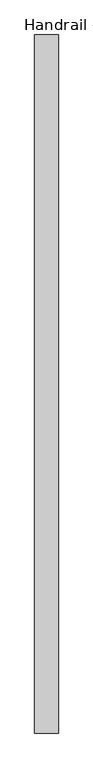
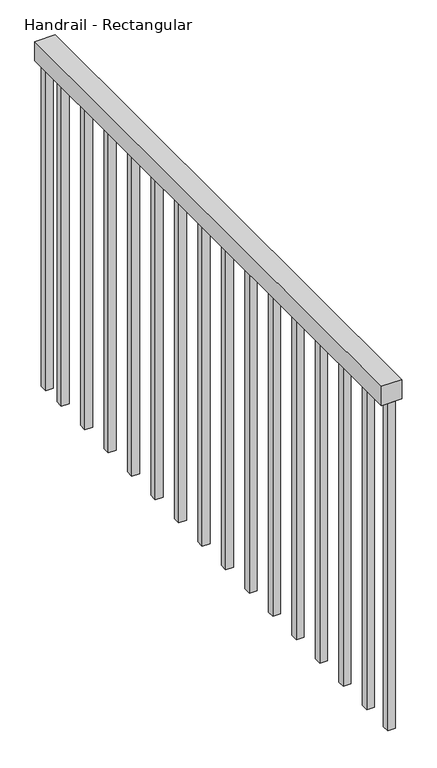
"""IFC4 building model written with IfcOpenShell, lengths in millimetres: railing geometry, Handrail - Rectangular."""

from ifc_helpers import new_model, si_unit, frame, origin, place, context, project, spatial, polyline, outline, extrude, source, transform, mapped, element, save


def handrail_rectangular_a0f4db76(model_context):
    return source(origin(), model_context, "Body", "SweptSolid", [
        extrude(outline(polyline([(-12364.4211091, 3845.8507146), (-12415.2211091, 3845.8507146), (-12415.2211091, 5345.8507146), (-12364.4211091, 5345.8507146), (-12364.4211091, 3845.8507146)])), frame((0.0, 0.0, 6654.4), z_axis=(0.0, 0.0, 1.0), x_axis=(1.0, 0.0, 0.0)), (0.0, 0.0, 1.0), 50.8),
        extrude(outline(polyline([(-12380.2961091, 5258.7257146), (-12399.3461091, 5258.7257146), (-12399.3461091, 5277.7757146), (-12380.2961091, 5277.7757146), (-12380.2961091, 5258.7257146)])), frame((0.0, 0.0, 5790.8), z_axis=(0.0, 0.0, 1.0), x_axis=(1.0, 0.0, 0.0)), (0.0, 0.0, 1.0), 863.6),
        extrude(outline(polyline([(-12380.2961091, 5157.1257146), (-12399.3461091, 5157.1257146), (-12399.3461091, 5176.1757146), (-12380.2961091, 5176.1757146), (-12380.2961091, 5157.1257146)])), frame((0.0, 0.0, 5790.8), z_axis=(0.0, 0.0, 1.0), x_axis=(1.0, 0.0, 0.0)), (0.0, 0.0, 1.0), 863.6),
        extrude(outline(polyline([(-12380.2961091, 5055.5257146), (-12399.3461091, 5055.5257146), (-12399.3461091, 5074.5757146), (-12380.2961091, 5074.5757146), (-12380.2961091, 5055.5257146)])), frame((0.0, 0.0, 5790.8), z_axis=(0.0, 0.0, 1.0), x_axis=(1.0, 0.0, 0.0)), (0.0, 0.0, 1.0), 863.6),
        extrude(outline(polyline([(-12380.2961091, 4953.9257146), (-12399.3461091, 4953.9257146), (-12399.3461091, 4972.9757146), (-12380.2961091, 4972.9757146), (-12380.2961091, 4953.9257146)])), frame((0.0, 0.0, 5790.8), z_axis=(0.0, 0.0, 1.0), x_axis=(1.0, 0.0, 0.0)), (0.0, 0.0, 1.0), 863.6),
        extrude(outline(polyline([(-12380.2961091, 4852.3257146), (-12399.3461091, 4852.3257146), (-12399.3461091, 4871.3757146), (-12380.2961091, 4871.3757146), (-12380.2961091, 4852.3257146)])), frame((0.0, 0.0, 5790.8), z_axis=(0.0, 0.0, 1.0), x_axis=(1.0, 0.0, 0.0)), (0.0, 0.0, 1.0), 863.6),
        extrude(outline(polyline([(-12380.2961091, 4750.7257146), (-12399.3461091, 4750.7257146), (-12399.3461091, 4769.7757146), (-12380.2961091, 4769.7757146), (-12380.2961091, 4750.7257146)])), frame((0.0, 0.0, 5790.8), z_axis=(0.0, 0.0, 1.0), x_axis=(1.0, 0.0, 0.0)), (0.0, 0.0, 1.0), 863.6),
        extrude(outline(polyline([(-12380.2961091, 4649.1257146), (-12399.3461091, 4649.1257146), (-12399.3461091, 4668.1757146), (-12380.2961091, 4668.1757146), (-12380.2961091, 4649.1257146)])), frame((0.0, 0.0, 5790.8), z_axis=(0.0, 0.0, 1.0), x_axis=(1.0, 0.0, 0.0)), (0.0, 0.0, 1.0), 863.6),
        extrude(outline(polyline([(-12380.2961091, 4547.5257146), (-12399.3461091, 4547.5257146), (-12399.3461091, 4566.5757146), (-12380.2961091, 4566.5757146), (-12380.2961091, 4547.5257146)])), frame((0.0, 0.0, 5790.8), z_axis=(0.0, 0.0, 1.0), x_axis=(1.0, 0.0, 0.0)), (0.0, 0.0, 1.0), 863.6),
        extrude(outline(polyline([(-12380.2961091, 4445.9257146), (-12399.3461091, 4445.9257146), (-12399.3461091, 4464.9757146), (-12380.2961091, 4464.9757146), (-12380.2961091, 4445.9257146)])), frame((0.0, 0.0, 5790.8), z_axis=(0.0, 0.0, 1.0), x_axis=(1.0, 0.0, 0.0)), (0.0, 0.0, 1.0), 863.6),
        extrude(outline(polyline([(-12380.2961091, 4344.3257146), (-12399.3461091, 4344.3257146), (-12399.3461091, 4363.3757146), (-12380.2961091, 4363.3757146), (-12380.2961091, 4344.3257146)])), frame((0.0, 0.0, 5790.8), z_axis=(0.0, 0.0, 1.0), x_axis=(1.0, 0.0, 0.0)), (0.0, 0.0, 1.0), 863.6),
        extrude(outline(polyline([(-12380.2961091, 4242.7257146), (-12399.3461091, 4242.7257146), (-12399.3461091, 4261.7757146), (-12380.2961091, 4261.7757146), (-12380.2961091, 4242.7257146)])), frame((0.0, 0.0, 5790.8), z_axis=(0.0, 0.0, 1.0), x_axis=(1.0, 0.0, 0.0)), (0.0, 0.0, 1.0), 863.6),
        extrude(outline(polyline([(-12380.2961091, 4141.1257146), (-12399.3461091, 4141.1257146), (-12399.3461091, 4160.1757146), (-12380.2961091, 4160.1757146), (-12380.2961091, 4141.1257146)])), frame((0.0, 0.0, 5790.8), z_axis=(0.0, 0.0, 1.0), x_axis=(1.0, 0.0, 0.0)), (0.0, 0.0, 1.0), 863.6),
        extrude(outline(polyline([(-12380.2961091, 4039.5257146), (-12399.3461091, 4039.5257146), (-12399.3461091, 4058.5757146), (-12380.2961091, 4058.5757146), (-12380.2961091, 4039.5257146)])), frame((0.0, 0.0, 5790.8), z_axis=(0.0, 0.0, 1.0), x_axis=(1.0, 0.0, 0.0)), (0.0, 0.0, 1.0), 863.6),
        extrude(outline(polyline([(-12380.2961091, 3937.9257146), (-12399.3461091, 3937.9257146), (-12399.3461091, 3956.9757146), (-12380.2961091, 3956.9757146), (-12380.2961091, 3937.9257146)])), frame((0.0, 0.0, 5790.8), z_axis=(0.0, 0.0, 1.0), x_axis=(1.0, 0.0, 0.0)), (0.0, 0.0, 1.0), 863.6),
        extrude(outline(polyline([(-12380.2961091, 5326.8007146), (-12399.3461091, 5326.8007146), (-12399.3461091, 5345.8507146), (-12380.2961091, 5345.8507146), (-12380.2961091, 5326.8007146)])), frame((0.0, 0.0, 5790.8), z_axis=(0.0, 0.0, 1.0), x_axis=(1.0, 0.0, 0.0)), (0.0, 0.0, 1.0), 863.6),
        extrude(outline(polyline([(-12380.2961091, 3845.8507146), (-12399.3461091, 3845.8507146), (-12399.3461091, 3864.9007146), (-12380.2961091, 3864.9007146), (-12380.2961091, 3845.8507146)])), frame((0.0, 0.0, 5790.8), z_axis=(0.0, 0.0, 1.0), x_axis=(1.0, 0.0, 0.0)), (0.0, 0.0, 1.0), 863.6),
    ])


if __name__ == "__main__":
    model = new_model("IFC4")
    model_context = context("Model", 3, world=origin())
    ifc_project = project(units=[si_unit("LENGTHUNIT", "METRE", prefix="MILLI")], contexts=[model_context])
    site = spatial("IfcSite", under=ifc_project)
    building = spatial("IfcBuilding", under=site)
    placement = place(None, origin())
    handrail_rectangular_shape = handrail_rectangular_a0f4db76(model_context)
    element("IfcRailing", 1, ObjectType="Handrail - Rectangular", at=placement, inside=building, context=model_context, shape_type="MappedRepresentation", body=[
        mapped(handrail_rectangular_shape, transform((0.0, 0.0, 0.0), x_axis=(1.0, 0.0, 0.0), y_axis=(0.0, 1.0, 0.0), z_axis=(0.0, 0.0, 1.0))),
    ])
    save(model, "model.ifc")
